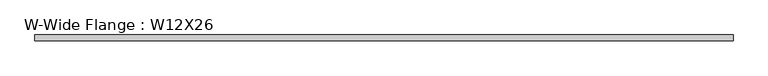
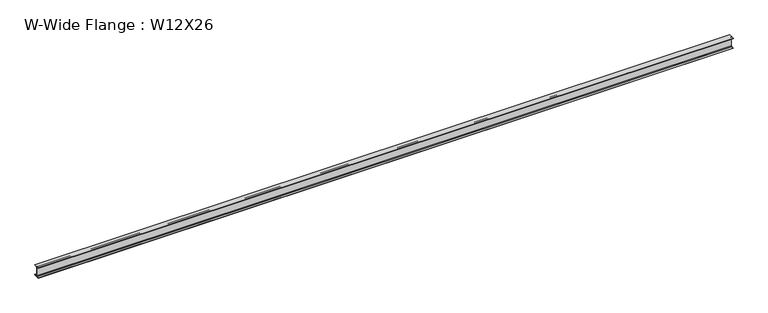
"""IFC4 building model written with IfcOpenShell, lengths in millimetres: beam geometry, W-Wide Flange : W12X26."""

from ifc_helpers import new_model, si_unit, point, frame, frame_2d, origin, place, context, project, spatial, polyline, circle_curve, trimmed, segment, composite_curve, outline, extrude, source, transform, mapped, element, save


def w_wide_flange_w12x26_0d1d3194(model_context):
    return source(origin(), model_context, "Body", "SweptSolid", [
        extrude(outline(composite_curve([segment(polyline([(82.4011719, -145.5539063), (82.4011719, -155.178125), (-82.4011719, -155.178125), (-82.4011719, -145.5539063), (-20.2902344, -145.5539063)]), True, "CONTINUOUS"), segment(trimmed(circle_curve(frame_2d((-20.2902344, -128.190625)), 17.3632812), [point((-20.2902344, -145.5539063))], [point((-2.9269531, -128.190625))], True, "CARTESIAN"), True, "CONTINUOUS"), segment(polyline([(-2.9269531, -128.190625), (-2.9269531, 128.190625)]), True, "CONTINUOUS"), segment(trimmed(circle_curve(frame_2d((-20.2902344, 128.190625)), 17.3632812), [point((-2.9269531, 128.190625))], [point((-20.2902344, 145.5539062))], True, "CARTESIAN"), True, "CONTINUOUS"), segment(polyline([(-20.2902344, 145.5539062), (-82.4011719, 145.5539062), (-82.4011719, 155.178125), (82.4011719, 155.178125), (82.4011719, 145.5539062), (20.2902344, 145.5539062)]), True, "CONTINUOUS"), segment(trimmed(circle_curve(frame_2d((20.2902344, 128.190625)), 17.3632812), [point((20.2902344, 145.5539062))], [point((2.9269531, 128.190625))], True, "CARTESIAN"), True, "CONTINUOUS"), segment(polyline([(2.9269531, 128.190625), (2.9269531, -128.190625)]), True, "CONTINUOUS"), segment(trimmed(circle_curve(frame_2d((20.2902344, -128.190625)), 17.3632812), [point((2.9269531, -128.190625))], [point((20.2902344, -145.5539063))], True, "CARTESIAN"), True, "CONTINUOUS"), segment(polyline([(20.2902344, -145.5539063), (82.4011719, -145.5539063)]), True, "CONTINUOUS")], self_intersect=False)), frame((-9946.48125, 0.0, 0.0), z_axis=(1.0, 0.0, 0.0), x_axis=(0.0, 1.0, 0.0)), (0.0, 0.0, 1.0), 19892.9625),
    ])


if __name__ == "__main__":
    model = new_model("IFC4")
    model_context = context("Model", 3, world=origin())
    ifc_project = project(units=[si_unit("LENGTHUNIT", "METRE", prefix="MILLI")], contexts=[model_context])
    site = spatial("IfcSite", under=ifc_project)
    building = spatial("IfcBuilding", under=site)
    placement = place(None, origin())
    w_wide_flange_w12x26_shape = w_wide_flange_w12x26_0d1d3194(model_context)
    element("IfcBeam", 1, ObjectType="W-Wide Flange : W12X26", at=placement, inside=building, context=model_context, shape_type="MappedRepresentation", body=[
        mapped(w_wide_flange_w12x26_shape, transform((0.0, 0.0, 0.0), x_axis=(1.0, 0.0, 0.0), y_axis=(0.0, 1.0, 0.0), z_axis=(0.0, 0.0, 1.0))),
    ])
    save(model, "model.ifc")

# Revit data of these elements
# Type "W-Wide Flange : W12X26"
#   Assembly Code = "B10"
#   W = 26
#   Length [instance default] = 5' - 0"
#   bf = 0' - 6 125/256"
#   d = 1' - 0 7/32"
#   k = 0' - 1 1/16"
#   k2 = 0' - 0 175/256"
#   tf = 0' - 0 97/256"
#   tw = 0' - 0 59/256"
#   A = 0.053125 SF
#   Structural Material [instance default] = none
# Element 1 (IfcBeam, "W-Wide Flange : W12X26")
#   Structural Material = Dark metal
#   Materials on its faces: "Dark metal"
# Materials
#   "Dark metal": class "Generic", colour RGB 44 29 29, transparency 0, Cost = 0
